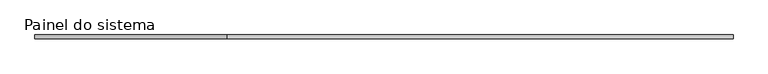
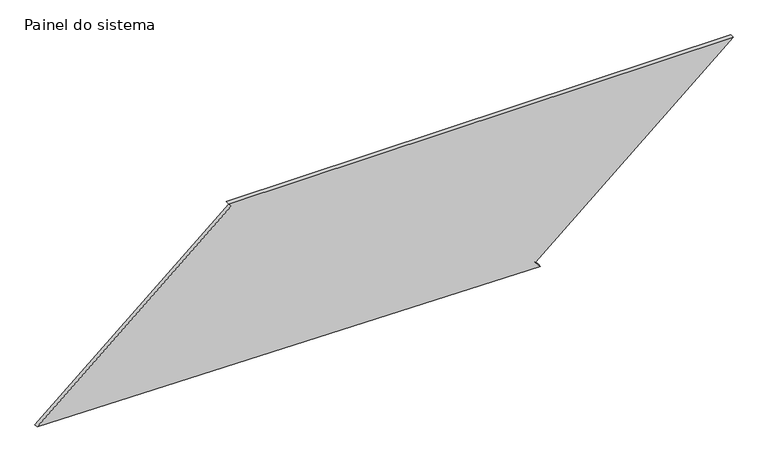
"""IFC4 building model written with IfcOpenShell, lengths in millimetres: plate geometry, Painel do sistema : Envidraçado."""

from ifc_helpers import new_model, si_unit, frame, origin, place, context, project, spatial, polyline, outline, extrude, source, transform, mapped, element, save


def painel_do_sistema_7f893fa8(model_context):
    return source(origin(), model_context, "Body", "SweptSolid", [
        extrude(outline(polyline([(0.0, 988.4736252), (38.0201724, 956.0010753), (1114.92065, 2216.879632), (1114.92065, -996.3809595), (1095.9105638, -980.1446846), (39.6308384, -2216.879632), (0.0, 988.4736252)])), frame((0.0, 24.5, 0.0), z_axis=(0.0, 1.0, 0.0), x_axis=(0.0, 0.0, 1.0)), (0.0, 0.0, 1.0), 25.0),
    ])


if __name__ == "__main__":
    model = new_model("IFC4")
    model_context = context("Model", 3, world=origin())
    ifc_project = project(units=[si_unit("LENGTHUNIT", "METRE", prefix="MILLI")], contexts=[model_context])
    site = spatial("IfcSite", under=ifc_project)
    building = spatial("IfcBuilding", under=site)
    placement = place(None, origin())
    painel_do_sistema_shape = painel_do_sistema_7f893fa8(model_context)
    element("IfcPlate", 1, ObjectType="Painel do sistema : Envidraçado", at=placement, inside=building, context=model_context, shape_type="MappedRepresentation", body=[
        mapped(painel_do_sistema_shape, transform((0.0, 0.0, 0.0), x_axis=(1.0, 0.0, 0.0), y_axis=(0.0, 1.0, 0.0), z_axis=(0.0, 0.0, 1.0))),
    ])
    save(model, "model.ifc")

# Revit data of these elements
# Type "Painel do sistema : Envidraçado"
#   Construction Type Id = "GSP4R"
#   Analytic Construction = "Vidraça única Pilkington 1/8 pol"
#   Visual Light Transmittance = 0.9
#   Solar Heat Gain Coefficient = 0.86
#   Heat Transfer Coefficient (U) = 6.7069 W/(m²·K)
# Element 1 (IfcPlate, "Painel do sistema : Envidraçado")
#   Materials on its faces: "Vidro"
# Materials
#   "Vidro": class "Vidro", colour RGB 0 128 192, transparency 0.9, Description = "Vidro de sílica", Cost = 0
